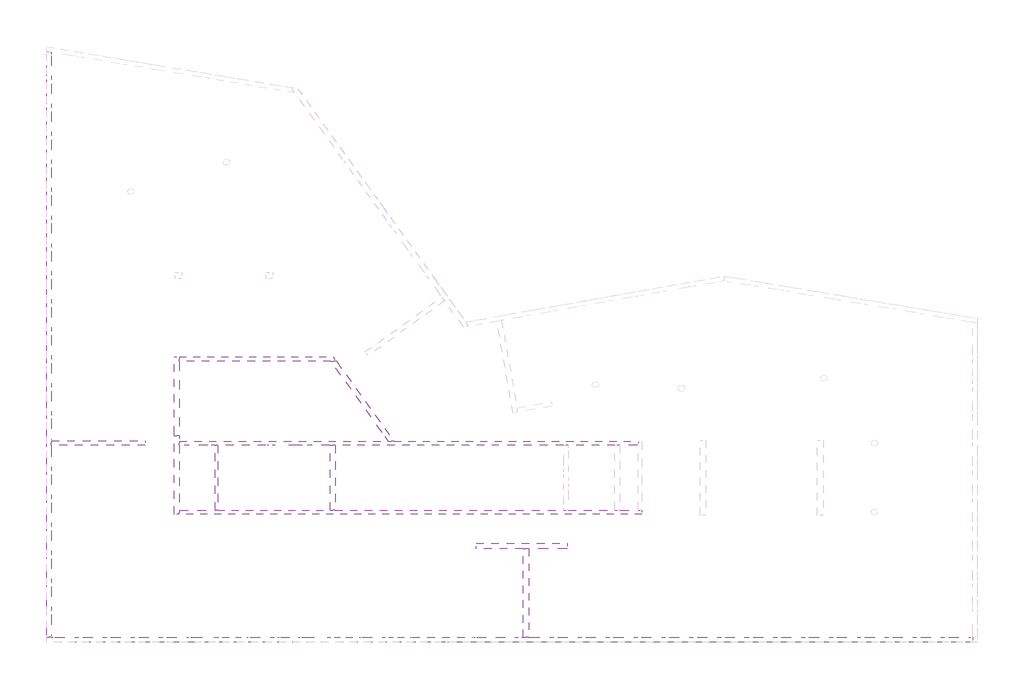
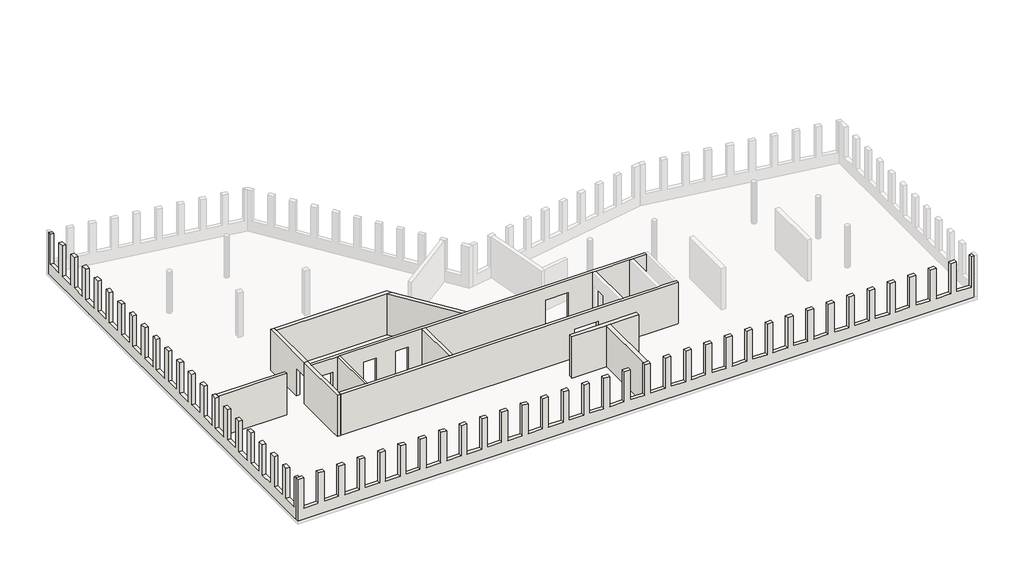
# One storey, part 1 of 2: 13 walls.
"""IFC4 building model written with IfcOpenShell, lengths in millimetres."""

from ifc_helpers import new_model, si_unit, frame, origin, place, context, project, spatial, polyline, outline, extrude, faceted_brep, element, save

model = new_model("IFC4")

# Units and contexts
model_context = context("Model", 3, world=origin())
ifc_project = project(units=[si_unit("LENGTHUNIT", "METRE", prefix="MILLI")], contexts=[model_context])

# Site, building, storey
site = spatial("IfcSite", under=ifc_project)
building = spatial("IfcBuilding", under=site)
storey = spatial("IfcBuildingStorey", under=building, Name="02_OG_OKFB_6,92", Elevation=6920.0)

# Walls
placement = place(None, origin())
element("IfcWall", 1, ObjectType="5dki Lochfassade 26cm C30/37", at=placement, inside=storey, context=model_context, shape_type="Brep", body=[
    faceted_brep([(49396.9999991, 130.0010483, 11090.0), (49396.9999991, 130.0010483, 13440.0), (49603.9991101, 130.0010486, 13440.0), (49603.9991101, 130.0010486, 10230.0), (25766.9999915, 130.0010117, 10230.0), (25466.9999915, 130.0010113, 10230.0), (130.0010047, 130.000972, 10230.0), (-129.9989953, 130.0009716, 10230.0), (-129.9989953, 130.0009716, 13440.0), (130.0010047, 130.000972, 13440.0), (317.0000012, 130.0009723, 13440.0), (316.999997, 130.0009723, 11090.0), (1397.0000012, 130.000974, 11090.0), (1397.0000069, 130.000974, 13440.0), (1816.9999991, 130.0009747, 13440.0), (1817.0000028, 130.0009747, 11090.0), (2896.9999991, 130.0009763, 11090.0), (2897.0000017, 130.0009763, 13440.0), (3316.9999991, 130.000977, 13440.0), (3316.9999977, 130.000977, 11090.0), (4396.9999991, 130.0009787, 11090.0), (4396.9999966, 130.0009787, 13440.0), (4816.9999991, 130.0009793, 13440.0), (4816.9999991, 130.0009793, 11090.0), (5896.9999991, 130.000981, 11090.0), (5896.9999991, 130.000981, 13440.0), (6316.9999991, 130.0009816, 13440.0), (6316.9999991, 130.0009816, 11090.0), (7396.9999991, 130.0009833, 11090.0), (7396.9999991, 130.0009833, 13440.0), (7816.9999991, 130.0009839, 13440.0), (7816.9999991, 130.0009839, 11090.0), (8896.9999991, 130.0009856, 11090.0), (8896.9999991, 130.0009856, 13440.0), (9316.9999991, 130.0009863, 13440.0), (9316.9999991, 130.0009863, 11090.0), (10396.9999991, 130.0009879, 11090.0), (10396.9999991, 130.0009879, 13440.0), (10816.9999991, 130.0009886, 13440.0), (10816.9999991, 130.0009886, 11090.0), (11896.9999991, 130.0009903, 11090.0), (11896.9999991, 130.0009903, 13440.0), (12316.9999991, 130.0009909, 13440.0), (12316.9999991, 130.0009909, 11090.0), (13396.9999991, 130.0009926, 11090.0), (13396.9999991, 130.0009926, 13440.0), (13816.9999991, 130.0009932, 13440.0), (13816.9999991, 130.0009932, 11090.0), (14896.9999991, 130.0009949, 11090.0), (14896.9999991, 130.0009949, 13440.0), (15316.9999991, 130.0009956, 13440.0), (15316.9999991, 130.0009956, 11090.0), (16396.9999991, 130.0009972, 11090.0), (16396.9999991, 130.0009972, 13440.0), (16816.9999991, 130.0009979, 13440.0), (16816.9999991, 130.0009979, 11090.0), (17896.9999991, 130.0009996, 11090.0), (17896.9999991, 130.0009996, 13440.0), (18316.9999991, 130.0010002, 13440.0), (18316.9999991, 130.0010002, 11090.0), (19396.9999991, 130.0010019, 11090.0), (19396.9999991, 130.0010019, 13440.0), (19816.9999991, 130.0010025, 13440.0), (19816.9999991, 130.0010025, 11090.0), (20896.9999991, 130.0010042, 11090.0), (20896.9999991, 130.0010042, 13440.0), (21316.9999991, 130.0010048, 13440.0), (21316.9999991, 130.0010048, 11090.0), (22396.9999991, 130.0010065, 11090.0), (22396.9999991, 130.0010065, 13440.0), (22816.9999991, 130.0010072, 13440.0), (22816.9999991, 130.0010072, 11090.0), (23896.9999991, 130.0010088, 11090.0), (23896.9999991, 130.0010088, 13440.0), (24316.9999991, 130.0010095, 13440.0), (24316.9999991, 130.0010095, 11090.0), (25396.9999991, 130.0010112, 11090.0), (25396.9999991, 130.0010112, 13440.0), (25466.9999915, 130.0010113, 13440.0), (25766.9999915, 130.0010117, 13440.0), (25816.9999991, 130.0010118, 13440.0), (25816.9999991, 130.0010118, 11090.0), (26896.9999991, 130.0010135, 11090.0), (26896.9999991, 130.0010135, 13440.0), (27316.9999991, 130.0010141, 13440.0), (27316.9999991, 130.0010141, 11090.0), (28396.9999991, 130.0010158, 11090.0), (28396.9999991, 130.0010158, 13440.0), (28816.9999991, 130.0010165, 13440.0), (28816.9999991, 130.0010165, 11090.0), (29896.9999991, 130.0010181, 11090.0), (29896.9999991, 130.0010181, 13440.0), (30316.9999991, 130.0010188, 13440.0), (30316.9999991, 130.0010188, 11090.0), (31396.9999991, 130.0010205, 11090.0), (31396.9999991, 130.0010205, 13440.0), (31816.9999991, 130.0010211, 13440.0), (31816.9999991, 130.0010211, 11090.0), (32896.9999991, 130.0010228, 11090.0), (32896.9999991, 130.0010228, 13440.0), (33316.9999991, 130.0010234, 13440.0), (33316.9999991, 130.0010234, 11090.0), (34396.9999991, 130.0010251, 11090.0), (34396.9999991, 130.0010251, 13440.0), (34816.9999991, 130.0010258, 13440.0), (34816.9999991, 130.0010258, 11090.0), (35896.9999991, 130.0010274, 11090.0), (35896.9999991, 130.0010274, 13440.0), (36316.9999991, 130.0010281, 13440.0), (36316.9999991, 130.0010281, 11090.0), (37396.9999991, 130.0010297, 11090.0), (37396.9999991, 130.0010297, 13440.0), (37816.9999991, 130.0010304, 13440.0), (37816.9999991, 130.0010304, 11090.0), (38896.9999991, 130.0010321, 11090.0), (38896.9999991, 130.0010321, 13440.0), (39316.9999991, 130.0010327, 13440.0), (39316.9999991, 130.0010327, 11090.0), (40396.9999991, 130.0010344, 11090.0), (40396.9999991, 130.0010344, 13440.0), (40816.9999991, 130.001035, 13440.0), (40816.9999991, 130.001035, 11090.0), (41896.9999991, 130.0010367, 11090.0), (41896.9999991, 130.0010367, 13440.0), (42316.9999991, 130.0010374, 13440.0), (42316.9999991, 130.0010374, 11090.0), (43396.9999991, 130.001039, 11090.0), (43396.9999991, 130.001039, 13440.0), (43816.9999991, 130.0010397, 13440.0), (43816.9999991, 130.0010397, 11090.0), (44896.9999991, 130.0010414, 11090.0), (44896.9999991, 130.0010414, 13440.0), (45316.9999991, 130.001042, 13440.0), (45316.9999991, 130.001042, 11090.0), (46396.9999991, 130.0010437, 11090.0), (46396.9999991, 130.0010437, 13440.0), (46816.9999991, 130.0010443, 13440.0), (46816.9999991, 130.0010443, 11090.0), (47896.9999991, 130.001046, 11090.0), (47896.9999991, 130.001046, 13440.0), (48316.9999991, 130.0010467, 13440.0), (48316.9999991, 130.0010467, 11090.0), (49603.9991105, -129.9989514, 13440.0), (49396.9999995, -129.9989517, 13440.0), (49396.9999995, -129.9989517, 11090.0), (48316.9999995, -129.9989533, 11090.0), (48316.9999995, -129.9989533, 13440.0), (47896.9999995, -129.998954, 13440.0), (47896.9999995, -129.998954, 11090.0), (46816.9999995, -129.9989557, 11090.0), (46816.9999995, -129.9989557, 13440.0), (46396.9999995, -129.9989563, 13440.0), (46396.9999995, -129.9989563, 11090.0), (45316.9999995, -129.998958, 11090.0), (45316.9999995, -129.998958, 13440.0), (44896.9999995, -129.9989586, 13440.0), (44896.9999995, -129.9989586, 11090.0), (43816.9999995, -129.9989603, 11090.0), (43816.9999995, -129.9989603, 13440.0), (43396.9999995, -129.998961, 13440.0), (43396.9999995, -129.998961, 11090.0), (42316.9999995, -129.9989626, 11090.0), (42316.9999995, -129.9989626, 13440.0), (41896.9999995, -129.9989633, 13440.0), (41896.9999995, -129.9989633, 11090.0), (40816.9999995, -129.998965, 11090.0), (40816.9999995, -129.998965, 13440.0), (40396.9999995, -129.9989656, 13440.0), (40396.9999995, -129.9989656, 11090.0), (39316.9999995, -129.9989673, 11090.0), (39316.9999995, -129.9989673, 13440.0), (38896.9999995, -129.9989679, 13440.0), (38896.9999995, -129.9989679, 11090.0), (37816.9999995, -129.9989696, 11090.0), (37816.9999995, -129.9989696, 13440.0), (37396.9999995, -129.9989703, 13440.0), (37396.9999995, -129.9989703, 11090.0), (36316.9999995, -129.9989719, 11090.0), (36316.9999995, -129.9989719, 13440.0), (35896.9999995, -129.9989726, 13440.0), (35896.9999995, -129.9989726, 11090.0), (34816.9999995, -129.9989742, 11090.0), (34816.9999995, -129.9989742, 13440.0), (34396.9999995, -129.9989749, 13440.0), (34396.9999995, -129.9989749, 11090.0), (33316.9999995, -129.9989766, 11090.0), (33316.9999995, -129.9989766, 13440.0), (32896.9999995, -129.9989772, 13440.0), (32896.9999995, -129.9989772, 11090.0), (31816.9999995, -129.9989789, 11090.0), (31816.9999995, -129.9989789, 13440.0), (31396.9999995, -129.9989795, 13440.0), (31396.9999995, -129.9989795, 11090.0), (30316.9999995, -129.9989812, 11090.0), (30316.9999995, -129.9989812, 13440.0), (29896.9999995, -129.9989819, 13440.0), (29896.9999995, -129.9989819, 11090.0), (28816.9999995, -129.9989835, 11090.0), (28816.9999995, -129.9989835, 13440.0), (28396.9999995, -129.9989842, 13440.0), (28396.9999995, -129.9989842, 11090.0), (27316.9999995, -129.9989859, 11090.0), (27316.9999995, -129.9989859, 13440.0), (26896.9999995, -129.9989865, 13440.0), (26896.9999995, -129.9989865, 11090.0), (25816.9999995, -129.9989882, 11090.0), (25816.9999995, -129.9989882, 13440.0), (25396.9999995, -129.9989888, 13440.0), (25396.9999995, -129.9989888, 11090.0), (24316.9999995, -129.9989905, 11090.0), (24316.9999995, -129.9989905, 13440.0), (23896.9999995, -129.9989912, 13440.0), (23896.9999995, -129.9989912, 11090.0), (22816.9999995, -129.9989928, 11090.0), (22816.9999995, -129.9989928, 13440.0), (22396.9999995, -129.9989935, 13440.0), (22396.9999995, -129.9989935, 11090.0), (21316.9999995, -129.9989952, 11090.0), (21316.9999995, -129.9989952, 13440.0), (20896.9999995, -129.9989958, 13440.0), (20896.9999995, -129.9989958, 11090.0), (19816.9999995, -129.9989975, 11090.0), (19816.9999995, -129.9989975, 13440.0), (19396.9999995, -129.9989981, 13440.0), (19396.9999995, -129.9989981, 11090.0), (18316.9999995, -129.9989998, 11090.0), (18316.9999995, -129.9989998, 13440.0), (17896.9999995, -129.9990004, 13440.0), (17896.9999995, -129.9990004, 11090.0), (16816.9999995, -129.9990021, 11090.0), (16816.9999995, -129.9990021, 13440.0), (16396.9999995, -129.9990028, 13440.0), (16396.9999995, -129.9990028, 11090.0), (15316.9999995, -129.9990044, 11090.0), (15316.9999995, -129.9990044, 13440.0), (14896.9999995, -129.9990051, 13440.0), (14896.9999995, -129.9990051, 11090.0), (13816.9999995, -129.9990068, 11090.0), (13816.9999995, -129.9990068, 13440.0), (13396.9999995, -129.9990074, 13440.0), (13396.9999995, -129.9990074, 11090.0), (12316.9999995, -129.9990091, 11090.0), (12316.9999995, -129.9990091, 13440.0), (11896.9999995, -129.9990097, 13440.0), (11896.9999995, -129.9990097, 11090.0), (10816.9999995, -129.9990114, 11090.0), (10816.9999995, -129.9990114, 13440.0), (10396.9999995, -129.9990121, 13440.0), (10396.9999995, -129.9990121, 11090.0), (9316.9999995, -129.9990137, 11090.0), (9316.9999995, -129.9990137, 13440.0), (8896.9999995, -129.9990144, 13440.0), (8896.9999995, -129.9990144, 11090.0), (7816.9999995, -129.9990161, 11090.0), (7816.9999995, -129.9990161, 13440.0), (7396.9999995, -129.9990167, 13440.0), (7396.9999995, -129.9990167, 11090.0), (6316.9999995, -129.9990184, 11090.0), (6316.9999995, -129.9990184, 13440.0), (5896.9999995, -129.999019, 13440.0), (5896.9999995, -129.999019, 11090.0), (4816.9999995, -129.9990207, 11090.0), (4816.9999995, -129.9990207, 13440.0), (4396.9999995, -129.9990213, 13440.0), (4396.9999966, -129.9990213, 11090.0), (3316.9999995, -129.999023, 11090.0), (3316.9999977, -129.999023, 13440.0), (2896.9999995, -129.9990237, 13440.0), (2897.0000017, -129.9990237, 11090.0), (1816.9999995, -129.9990253, 11090.0), (1817.0000028, -129.9990253, 13440.0), (1397.0000016, -129.999026, 13440.0), (1397.0000069, -129.999026, 11090.0), (317.0000016, -129.9990277, 11090.0), (316.999997, -129.9990277, 13440.0), (-129.9989953, -129.9990284, 13440.0), (-129.9989953, -129.9990284, 10230.0), (49603.9991105, -129.9989514, 10230.0)], [[[0, 1, 2, 3, 4, 5, 6, 7, 8, 9, 10, 11, 12, 13, 14, 15, 16, 17, 18, 19, 20, 21, 22, 23, 24, 25, 26, 27, 28, 29, 30, 31, 32, 33, 34, 35, 36, 37, 38, 39, 40, 41, 42, 43, 44, 45, 46, 47, 48, 49, 50, 51, 52, 53, 54, 55, 56, 57, 58, 59, 60, 61, 62, 63, 64, 65, 66, 67, 68, 69, 70, 71, 72, 73, 74, 75, 76, 77, 78, 79, 80, 81, 82, 83, 84, 85, 86, 87, 88, 89, 90, 91, 92, 93, 94, 95, 96, 97, 98, 99, 100, 101, 102, 103, 104, 105, 106, 107, 108, 109, 110, 111, 112, 113, 114, 115, 116, 117, 118, 119, 120, 121, 122, 123, 124, 125, 126, 127, 128, 129, 130, 131, 132, 133, 134, 135, 136, 137, 138, 139, 140, 141]], [[142, 143, 144, 145, 146, 147, 148, 149, 150, 151, 152, 153, 154, 155, 156, 157, 158, 159, 160, 161, 162, 163, 164, 165, 166, 167, 168, 169, 170, 171, 172, 173, 174, 175, 176, 177, 178, 179, 180, 181, 182, 183, 184, 185, 186, 187, 188, 189, 190, 191, 192, 193, 194, 195, 196, 197, 198, 199, 200, 201, 202, 203, 204, 205, 206, 207, 208, 209, 210, 211, 212, 213, 214, 215, 216, 217, 218, 219, 220, 221, 222, 223, 224, 225, 226, 227, 228, 229, 230, 231, 232, 233, 234, 235, 236, 237, 238, 239, 240, 241, 242, 243, 244, 245, 246, 247, 248, 249, 250, 251, 252, 253, 254, 255, 256, 257, 258, 259, 260, 261, 262, 263, 264, 265, 266, 267, 268, 269, 270, 271, 272, 273, 274, 275, 276, 277]], [[7, 6, 5, 4, 3, 277, 276]], [[17, 267, 266, 18]], [[270, 14, 13, 271]], [[263, 262, 22, 21]], [[259, 258, 26, 25]], [[255, 254, 30, 29]], [[251, 250, 34, 33]], [[247, 246, 38, 37]], [[243, 242, 42, 41]], [[239, 238, 46, 45]], [[235, 234, 50, 49]], [[231, 230, 54, 53]], [[227, 226, 58, 57]], [[223, 222, 62, 61]], [[219, 218, 66, 65]], [[215, 214, 70, 69]], [[211, 210, 74, 73]], [[207, 206, 80, 79, 78, 77]], [[203, 202, 84, 83]], [[199, 198, 88, 87]], [[195, 194, 92, 91]], [[191, 190, 96, 95]], [[187, 186, 100, 99]], [[183, 182, 104, 103]], [[179, 178, 108, 107]], [[175, 174, 112, 111]], [[171, 170, 116, 115]], [[167, 166, 120, 119]], [[163, 162, 124, 123]], [[159, 158, 128, 127]], [[155, 154, 132, 131]], [[151, 150, 136, 135]], [[140, 139, 147, 146]], [[2, 1, 143, 142]], [[10, 9, 8, 275, 274]], [[3, 2, 142, 277]], [[12, 272, 271, 13]], [[273, 11, 10, 274]], [[272, 12, 11, 273]], [[16, 268, 267, 17]], [[269, 15, 14, 270]], [[268, 16, 15, 269]], [[20, 264, 263, 21]], [[265, 19, 18, 266]], [[264, 20, 19, 265]], [[25, 24, 260, 259]], [[23, 22, 262, 261]], [[24, 23, 261, 260]], [[29, 28, 256, 255]], [[27, 26, 258, 257]], [[28, 27, 257, 256]], [[33, 32, 252, 251]], [[31, 30, 254, 253]], [[32, 31, 253, 252]], [[37, 36, 248, 247]], [[35, 34, 250, 249]], [[36, 35, 249, 248]], [[41, 40, 244, 243]], [[39, 38, 246, 245]], [[40, 39, 245, 244]], [[45, 44, 240, 239]], [[43, 42, 242, 241]], [[44, 43, 241, 240]], [[49, 48, 236, 235]], [[47, 46, 238, 237]], [[48, 47, 237, 236]], [[53, 52, 232, 231]], [[51, 50, 234, 233]], [[52, 51, 233, 232]], [[57, 56, 228, 227]], [[55, 54, 230, 229]], [[56, 55, 229, 228]], [[61, 60, 224, 223]], [[59, 58, 226, 225]], [[60, 59, 225, 224]], [[65, 64, 220, 219]], [[63, 62, 222, 221]], [[64, 63, 221, 220]], [[69, 68, 216, 215]], [[67, 66, 218, 217]], [[68, 67, 217, 216]], [[73, 72, 212, 211]], [[71, 70, 214, 213]], [[72, 71, 213, 212]], [[77, 76, 208, 207]], [[75, 74, 210, 209]], [[76, 75, 209, 208]], [[83, 82, 204, 203]], [[81, 80, 206, 205]], [[82, 81, 205, 204]], [[87, 86, 200, 199]], [[85, 84, 202, 201]], [[86, 85, 201, 200]], [[91, 90, 196, 195]], [[89, 88, 198, 197]], [[90, 89, 197, 196]], [[95, 94, 192, 191]], [[93, 92, 194, 193]], [[94, 93, 193, 192]], [[99, 98, 188, 187]], [[97, 96, 190, 189]], [[98, 97, 189, 188]], [[103, 102, 184, 183]], [[101, 100, 186, 185]], [[102, 101, 185, 184]], [[107, 106, 180, 179]], [[105, 104, 182, 181]], [[106, 105, 181, 180]], [[111, 110, 176, 175]], [[109, 108, 178, 177]], [[110, 109, 177, 176]], [[115, 114, 172, 171]], [[113, 112, 174, 173]], [[114, 113, 173, 172]], [[119, 118, 168, 167]], [[117, 116, 170, 169]], [[118, 117, 169, 168]], [[123, 122, 164, 163]], [[121, 120, 166, 165]], [[122, 121, 165, 164]], [[127, 126, 160, 159]], [[125, 124, 162, 161]], [[126, 125, 161, 160]], [[131, 130, 156, 155]], [[129, 128, 158, 157]], [[130, 129, 157, 156]], [[135, 134, 152, 151]], [[133, 132, 154, 153]], [[134, 133, 153, 152]], [[139, 138, 148, 147]], [[137, 136, 150, 149]], [[138, 137, 149, 148]], [[146, 145, 141, 140]], [[144, 143, 1, 0]], [[145, 144, 0, 141]], [[8, 7, 276, 275]]]),
])
element("IfcWall", 2, ObjectType="5dki STB-Wand Kern 25cm C30/37", at=placement, inside=storey, context=model_context, shape_type="Brep", body=[
    faceted_brep([(6989.9999766, 15192.0124447, 13440.0), (6989.9999766, 14942.0124447, 13440.0), (6989.9999766, 10947.0136187, 13440.0), (6989.9999766, 10947.0136187, 12365.0), (6989.9999766, 11957.013616, 12365.0), (6989.9999766, 11957.013616, 10230.0), (6989.9999766, 14942.0124447, 10230.0), (6989.9999766, 15192.0124447, 10230.0), (6739.9999766, 10947.0136187, 13440.0), (6739.9999766, 15192.0124447, 13440.0), (6739.9999766, 15192.0124447, 10230.0), (6739.9999766, 11957.013616, 10230.0), (6739.9999766, 11957.013616, 12365.0), (6739.9999766, 10947.0136187, 12365.0)], [[[0, 1, 2, 3, 4, 5, 6, 7]], [[8, 9, 10, 11, 12, 13]], [[10, 7, 6, 5, 11]], [[2, 1, 0, 9, 8]], [[2, 8, 13, 3]], [[0, 7, 10, 9]], [[4, 12, 11, 5]], [[12, 4, 3, 13]]]),
])
element("IfcWall", 3, ObjectType="5dki STB-Wand Kern 25cm C30/37", at=placement, inside=storey, context=model_context, shape_type="Brep", body=[
    faceted_brep([(6989.9999766, 14942.0124447, 10230.0), (15141.8279932, 14942.0124447, 10230.0), (15449.8792779, 14942.0124447, 10230.0), (15449.8792779, 14942.0124447, 13440.0), (15141.8279932, 14942.0124447, 13440.0), (6989.9999766, 14942.0124447, 13440.0), (6989.9999766, 15192.0124447, 10230.0), (6989.9999766, 15192.0124447, 13440.0), (15269.8915173, 15192.0124447, 13440.0), (15269.8915173, 15192.0124447, 10230.0)], [[[0, 1, 2, 3, 4, 5]], [[6, 7, 8, 9]], [[2, 1, 0, 6, 9]], [[5, 4, 3, 8, 7]], [[0, 5, 7, 6]], [[3, 2, 9, 8]]]),
])
element("IfcWall", 4, ObjectType="5dki STB-Wand Kern 25cm C30/37", at=placement, inside=storey, context=model_context, shape_type="Brep", body=[
    faceted_brep([(18223.2182524, 10662.0127257, 13440.0), (15141.8279932, 14942.0124447, 13440.0), (15141.8279932, 14942.0124447, 10230.0), (17305.3310134, 11936.9428041, 10230.0), (17305.3310134, 11936.9428041, 12365.0), (17895.4523577, 11117.2740911, 12365.0), (17895.4523577, 11117.2740911, 10230.0), (18223.2182524, 10662.0127257, 10230.0), (15449.8792779, 14942.0124447, 13440.0), (18531.2695366, 10662.0127262, 13440.0), (18531.2695366, 10662.0127262, 10230.0), (18098.340653, 11263.3437308, 10230.0), (18098.340653, 11263.3437308, 12365.0), (17508.2193087, 12083.0124438, 12365.0), (17508.2193087, 12083.0124438, 10230.0), (15449.8792779, 14942.0124447, 10230.0)], [[[0, 1, 2, 3, 4, 5, 6, 7]], [[8, 9, 10, 11, 12, 13, 14, 15]], [[2, 15, 14, 3]], [[10, 7, 6, 11]], [[1, 0, 9, 8]], [[2, 1, 8, 15]], [[0, 7, 10, 9]], [[13, 4, 3, 14]], [[4, 13, 12, 5]], [[5, 12, 11, 6]]]),
])
element("IfcWall", 5, ObjectType="5dki STB-Wand Kern 25cm C30/37", at=placement, inside=storey, context=model_context, shape_type="Brep", body=[
    faceted_brep([(6739.9995723, 10947.0136187, 10230.0), (6739.9995723, 6740.0000204, 10230.0), (6739.9995723, 6740.0000204, 13440.0), (6739.9995723, 10947.0136187, 13440.0), (6739.9995723, 10947.0136187, 12365.0), (6989.9995723, 10947.0136187, 10230.0), (6989.9995723, 10947.0136187, 12365.0), (6989.9995723, 10947.0136187, 13440.0), (6989.9995723, 10662.0127052, 13440.0), (6989.9995723, 10442.0127052, 13440.0), (6989.9995723, 6960.0000208, 13440.0), (6989.9995723, 6740.0000208, 13440.0), (6989.9995723, 6740.0000208, 10230.0), (6989.9995723, 6960.0000208, 10230.0), (6989.9995723, 10442.0127052, 10230.0), (6989.9995723, 10662.0127052, 10230.0)], [[[0, 1, 2, 3, 4]], [[5, 6, 7, 8, 9, 10, 11, 12, 13, 14, 15]], [[1, 0, 5, 15, 14, 13, 12]], [[3, 2, 11, 10, 9, 8, 7]], [[0, 4, 3, 7, 6, 5]], [[2, 1, 12, 11]]]),
])
element("IfcWall", 6, ObjectType="5dki STB-Wand Kern 22cm C30/37", at=placement, inside=storey, context=model_context, shape_type="Brep", body=[
    faceted_brep([(31841.999935, 6740.0000516, 13440.0), (6989.9995723, 6740.0000208, 13440.0), (6989.9995723, 6740.0000208, 10230.0), (24166.9999591, 6740.0000421, 10230.0), (24166.999888, 6740.0000421, 12490.0), (25926.9999591, 6740.0000443, 12490.0), (25927.000338, 6740.0000443, 10230.0), (31841.999935, 6740.0000516, 10230.0), (6989.9995723, 6960.0000208, 13440.0), (8916.9999886, 6960.0000232, 13440.0), (9066.9999886, 6960.0000233, 13440.0), (15117.0008797, 6960.0000309, 13440.0), (15367.0008797, 6960.0000312, 13440.0), (27641.9999886, 6960.0000464, 13440.0), (27891.9999886, 6960.0000467, 13440.0), (30391.9999891, 6960.0000498, 13440.0), (30641.9999891, 6960.0000501, 13440.0), (31641.9999382, 6960.0000514, 13440.0), (31841.9999382, 6960.0000516, 13440.0), (31841.9999382, 6960.0000516, 10230.0), (31641.9999382, 6960.0000514, 10230.0), (30641.9999891, 6960.0000501, 10230.0), (30391.9999891, 6960.0000498, 10230.0), (27891.9999886, 6960.0000467, 10230.0), (27641.9999886, 6960.0000464, 10230.0), (25926.9999588, 6960.0000443, 10230.0), (25927.000338, 6960.0000443, 12490.0), (24166.9999588, 6960.0000421, 12490.0), (24166.999888, 6960.0000421, 10230.0), (15367.0008797, 6960.0000312, 10230.0), (15117.0008797, 6960.0000309, 10230.0), (9066.9999886, 6960.0000233, 10230.0), (8916.9999886, 6960.0000232, 10230.0), (6989.9995723, 6960.0000208, 10230.0)], [[[0, 1, 2, 3, 4, 5, 6, 7]], [[8, 9, 10, 11, 12, 13, 14, 15, 16, 17, 18, 19, 20, 21, 22, 23, 24, 25, 26, 27, 28, 29, 30, 31, 32, 33]], [[2, 33, 32, 31, 30, 29, 28, 3]], [[19, 7, 6, 25, 24, 23, 22, 21, 20]], [[1, 0, 18, 17, 16, 15, 14, 13, 12, 11, 10, 9, 8]], [[2, 1, 8, 33]], [[0, 7, 19, 18]], [[5, 26, 25, 6]], [[26, 5, 4, 27]], [[27, 4, 3, 28]]]),
])
element("IfcWall", 7, ObjectType="5dki STB-Wand Kern 22cm C30/37", at=placement, inside=storey, context=model_context, shape_type="Brep", body=[
    faceted_brep([(6989.9995723, 10662.0127052, 13440.0), (18223.2182524, 10662.0127257, 13440.0), (18531.2695366, 10662.0127262, 13440.0), (31641.9999912, 10662.0127502, 13440.0), (31641.9999912, 10662.0127502, 10230.0), (25926.999945, 10662.0127397, 10230.0), (25927.0000254, 10662.0127397, 12490.0), (24166.999945, 10662.0127365, 12490.0), (24166.9998144, 10662.0127365, 10230.0), (18531.2695366, 10662.0127262, 10230.0), (18223.2182524, 10662.0127257, 10230.0), (14152.0004935, 10662.0127182, 10230.0), (14152.0007698, 10662.0127182, 12365.0), (13142.0004935, 10662.0127164, 12365.0), (13142.0009721, 10662.0127164, 10230.0), (11796.9999806, 10662.0127139, 10230.0), (11796.9997327, 10662.0127139, 12365.0), (10786.9999806, 10662.0127121, 12365.0), (10786.999935, 10662.0127121, 10230.0), (8540.0010342, 10662.012708, 10230.0), (8540.000485, 10662.012708, 12365.0), (7530.0010342, 10662.0127061, 12365.0), (7530.0006873, 10662.0127061, 10230.0), (6989.9995723, 10662.0127052, 10230.0), (31641.9999881, 10442.0127502, 13440.0), (30641.9999891, 10442.0127483, 13440.0), (30391.9999891, 10442.0127479, 13440.0), (27891.9999829, 10442.0127433, 13440.0), (27641.9999829, 10442.0127429, 13440.0), (15367.0008797, 10442.0127204, 13440.0), (15117.0008797, 10442.01272, 13440.0), (9066.9999886, 10442.0127089, 13440.0), (8916.9999886, 10442.0127087, 13440.0), (6989.9995723, 10442.0127052, 13440.0), (6989.9995723, 10442.0127052, 10230.0), (7530.0010346, 10442.0127061, 10230.0), (7530.0006873, 10442.0127061, 12365.0), (8540.0010346, 10442.012708, 12365.0), (8540.000485, 10442.012708, 10230.0), (8916.9999886, 10442.0127087, 10230.0), (9066.9999886, 10442.0127089, 10230.0), (10786.999981, 10442.0127121, 10230.0), (10786.999935, 10442.0127121, 12365.0), (11796.999981, 10442.0127139, 12365.0), (11796.9997327, 10442.0127139, 10230.0), (13142.0004939, 10442.0127164, 10230.0), (13142.0009721, 10442.0127164, 12365.0), (14152.0004939, 10442.0127182, 12365.0), (14152.0007698, 10442.0127182, 10230.0), (15117.0008797, 10442.01272, 10230.0), (15367.0008797, 10442.0127204, 10230.0), (24166.9999454, 10442.0127365, 10230.0), (24166.9998144, 10442.0127365, 12490.0), (25926.9999454, 10442.0127397, 12490.0), (25927.0000254, 10442.0127397, 10230.0), (27641.9999829, 10442.0127429, 10230.0), (27891.9999829, 10442.0127433, 10230.0), (30391.9999891, 10442.0127479, 10230.0), (30641.9999891, 10442.0127483, 10230.0), (31641.9999881, 10442.0127502, 10230.0)], [[[0, 1, 2, 3, 4, 5, 6, 7, 8, 9, 10, 11, 12, 13, 14, 15, 16, 17, 18, 19, 20, 21, 22, 23]], [[24, 25, 26, 27, 28, 29, 30, 31, 32, 33, 34, 35, 36, 37, 38, 39, 40, 41, 42, 43, 44, 45, 46, 47, 48, 49, 50, 51, 52, 53, 54, 55, 56, 57, 58, 59]], [[34, 23, 22, 35]], [[4, 59, 58, 57, 56, 55, 54, 5]], [[8, 51, 50, 49, 48, 11, 10, 9]], [[18, 41, 40, 39, 38, 19]], [[44, 15, 14, 45]], [[3, 2, 1, 0, 33, 32, 31, 30, 29, 28, 27, 26, 25, 24]], [[0, 23, 34, 33]], [[4, 3, 24, 59]], [[53, 6, 5, 54]], [[6, 53, 52, 7]], [[7, 52, 51, 8]], [[17, 42, 41, 18]], [[42, 17, 16, 43]], [[43, 16, 15, 44]], [[13, 46, 45, 14]], [[46, 13, 12, 47]], [[47, 12, 11, 48]], [[21, 36, 35, 22]], [[36, 21, 20, 37]], [[37, 20, 19, 38]]]),
])
element("IfcWall", 8, ObjectType="5dki STB-Wand Kern 25cm C30/37", at=placement, inside=storey, context=model_context, shape_type="SweptSolid", body=[
    extrude(outline(polyline([(15117.0008797, 6960.0000309), (15117.0008797, 10442.01272), (15367.0008797, 10442.0127204), (15367.0008797, 6960.0000312), (15117.0008797, 6960.0000309)])), frame((0.0, 0.0, 10230.0), z_axis=(0.0, 0.0, 1.0), x_axis=(1.0, 0.0, 0.0)), (0.0, 0.0, 1.0), 3210.0),
])
element("IfcWall", 9, ObjectType="5dki STB-Wand Kern 15cm C30/37", at=placement, inside=storey, context=model_context, shape_type="SweptSolid", body=[
    extrude(outline(polyline([(8916.9999886, 6960.0000232), (8916.9999886, 10442.0127087), (9066.9999886, 10442.0127089), (9066.9999886, 6960.0000233), (8916.9999886, 6960.0000232)])), frame((0.0, 0.0, 10230.0), z_axis=(0.0, 0.0, 1.0), x_axis=(1.0, 0.0, 0.0)), (0.0, 0.0, 1.0), 3210.0),
])
element("IfcWall", 10, ObjectType="5dki Lochfassade 26cm C30/37", at=placement, inside=storey, context=model_context, shape_type="Brep", body=[
    faceted_brep([(130.0010047, 24278.4322867, 11090.0), (130.0010047, 24278.4322867, 13440.0), (130.0010047, 23857.0124158, 13440.0), (130.0010047, 23857.0124158, 11090.0), (130.0010047, 22777.0124158, 11090.0), (130.0010047, 22777.0124158, 13440.0), (130.0010047, 22357.0124158, 13440.0), (130.0010047, 22357.0124158, 11090.0), (130.0010047, 21277.0124158, 11090.0), (130.0010047, 21277.0124158, 13440.0), (130.0010047, 20857.0124158, 13440.0), (130.0010047, 20857.0124158, 11090.0), (130.0010047, 19777.0124158, 11090.0), (130.0010047, 19777.0124158, 13440.0), (130.0010047, 19357.0124158, 13440.0), (130.0010047, 19357.0124158, 11090.0), (130.0010047, 18277.0124158, 11090.0), (130.0010047, 18277.0124158, 13440.0), (130.0010047, 17857.0124158, 13440.0), (130.0010047, 17857.0124158, 11090.0), (130.0010047, 16777.0124158, 11090.0), (130.0010047, 16777.0124158, 13440.0), (130.0010047, 16357.0124158, 13440.0), (130.0010047, 16357.0124158, 11090.0), (130.0010047, 15277.0124158, 11090.0), (130.0010047, 15277.0124158, 13440.0), (130.0010047, 14857.0124158, 13440.0), (130.0010047, 14857.0124158, 11090.0), (130.0010047, 13777.0124158, 11090.0), (130.0010047, 13777.0124158, 13440.0), (130.0010047, 13357.0124158, 13440.0), (130.0010047, 13357.0124158, 11090.0), (130.0010047, 12277.0124158, 11090.0), (130.0010047, 12277.0124158, 13440.0), (130.0010047, 11857.0124158, 13440.0), (130.0010047, 11857.0124158, 11090.0), (130.0010047, 10777.0124158, 11090.0), (130.0010047, 10777.0124158, 13440.0), (130.0010047, 10692.0124295, 13440.0), (130.0010047, 10442.0124295, 13440.0), (130.0010047, 10357.0124158, 13440.0), (130.0010047, 10357.0124158, 11090.0), (130.0010047, 9277.0124158, 11090.0), (130.0010047, 9277.0124158, 13440.0), (130.0010047, 8857.0124158, 13440.0), (130.0010047, 8857.0124158, 11090.0), (130.0010047, 7777.0124158, 11090.0), (130.0010047, 7777.0124158, 13440.0), (130.0010047, 7357.0124158, 13440.0), (130.0010047, 7357.0124158, 11090.0), (130.0010047, 6277.0124158, 11090.0), (130.0010047, 6277.0124158, 13440.0), (130.0010047, 5857.0124158, 13440.0), (130.0010047, 5857.0124158, 11090.0), (130.0010047, 4777.0124158, 11090.0), (130.0010047, 4777.0124158, 13440.0), (130.0010047, 4357.0124158, 13440.0), (130.0010047, 4357.0124158, 11090.0), (130.0010047, 3277.0124158, 11090.0), (130.0010047, 3277.0124158, 13440.0), (130.0010047, 2857.0124158, 13440.0), (130.0010047, 2857.0124158, 11090.0), (130.0010047, 1777.0124158, 11090.0), (130.0010047, 1777.0124158, 13440.0), (130.0010047, 1357.0124158, 13440.0), (130.0010047, 1357.0124158, 11090.0), (130.0010047, 277.0124158, 11090.0), (130.0010047, 277.0124158, 13440.0), (130.0010047, 130.000972, 13440.0), (130.0010047, 130.000972, 10230.0), (130.0010047, 10442.0124295, 10230.0), (130.0010047, 10692.0124295, 10230.0), (130.0010047, 31548.6978518, 10230.0), (130.0010047, 31548.6978518, 13440.0), (130.0010047, 31357.0124158, 13440.0), (130.0010047, 31357.0124158, 11090.0), (130.0010047, 30277.0124158, 11090.0), (130.0010047, 30277.0124158, 13440.0), (130.0010047, 29857.0124158, 13440.0), (130.0010047, 29857.0124158, 11090.0), (130.0010047, 28777.0124158, 11090.0), (130.0010047, 28777.0124158, 13440.0), (130.0010047, 28358.4322867, 13440.0), (130.0010047, 28358.4322867, 11090.0), (130.0010047, 27278.4322867, 11090.0), (130.0010047, 27278.4322867, 13440.0), (130.0010047, 26858.4322867, 13440.0), (130.0010047, 26858.4322867, 11090.0), (130.0010047, 25778.4322867, 11090.0), (130.0010047, 25778.4322867, 13440.0), (130.0010047, 25358.4322867, 13440.0), (130.0010047, 25358.4322867, 11090.0), (-129.9989953, 23857.0124158, 13440.0), (-129.9989953, 24278.4322867, 13440.0), (-129.9989953, 24278.4322867, 11090.0), (-129.9989953, 25358.4322867, 11090.0), (-129.9989953, 25358.4322867, 13440.0), (-129.9989953, 25778.4322867, 13440.0), (-129.9989953, 25778.4322867, 11090.0), (-129.9989953, 26858.4322867, 11090.0), (-129.9989953, 26858.4322867, 13440.0), (-129.9989953, 27278.4322867, 13440.0), (-129.9989953, 27278.4322867, 11090.0), (-129.9989953, 28358.4322867, 11090.0), (-129.9989953, 28358.4322867, 13440.0), (-129.9989953, 28777.0124158, 13440.0), (-129.9989953, 28777.0124158, 11090.0), (-129.9989953, 29857.0124158, 11090.0), (-129.9989953, 29857.0124158, 13440.0), (-129.9989953, 30277.0124158, 13440.0), (-129.9989953, 30277.0124158, 11090.0), (-129.9989953, 31357.0124158, 11090.0), (-129.9989953, 31357.0124158, 13440.0), (-129.9989953, 31592.114918, 13440.0), (-129.9989953, 31592.114918, 10230.0), (-129.9989953, 130.0009716, 10230.0), (-129.9989953, 130.0009716, 13440.0), (-129.9989953, 277.0124158, 13440.0), (-129.9989953, 277.0124158, 11090.0), (-129.9989953, 1357.0124158, 11090.0), (-129.9989953, 1357.0124158, 13440.0), (-129.9989953, 1777.0124158, 13440.0), (-129.9989953, 1777.0124158, 11090.0), (-129.9989953, 2857.0124158, 11090.0), (-129.9989953, 2857.0124158, 13440.0), (-129.9989953, 3277.0124158, 13440.0), (-129.9989953, 3277.0124158, 11090.0), (-129.9989953, 4357.0124158, 11090.0), (-129.9989953, 4357.0124158, 13440.0), (-129.9989953, 4777.0124158, 13440.0), (-129.9989953, 4777.0124158, 11090.0), (-129.9989953, 5857.0124158, 11090.0), (-129.9989953, 5857.0124158, 13440.0), (-129.9989953, 6277.0124158, 13440.0), (-129.9989953, 6277.0124158, 11090.0), (-129.9989953, 7357.0124158, 11090.0), (-129.9989953, 7357.0124158, 13440.0), (-129.9989953, 7777.0124158, 13440.0), (-129.9989953, 7777.0124158, 11090.0), (-129.9989953, 8857.0124158, 11090.0), (-129.9989953, 8857.0124158, 13440.0), (-129.9989953, 9277.0124158, 13440.0), (-129.9989953, 9277.0124158, 11090.0), (-129.9989953, 10357.0124158, 11090.0), (-129.9989953, 10357.0124158, 13440.0), (-129.9989953, 10777.0124158, 13440.0), (-129.9989953, 10777.0124158, 11090.0), (-129.9989953, 11857.0124158, 11090.0), (-129.9989953, 11857.0124158, 13440.0), (-129.9989953, 12277.0124158, 13440.0), (-129.9989953, 12277.0124158, 11090.0), (-129.9989953, 13357.0124158, 11090.0), (-129.9989953, 13357.0124158, 13440.0), (-129.9989953, 13777.0124158, 13440.0), (-129.9989953, 13777.0124158, 11090.0), (-129.9989953, 14857.0124158, 11090.0), (-129.9989953, 14857.0124158, 13440.0), (-129.9989953, 15277.0124158, 13440.0), (-129.9989953, 15277.0124158, 11090.0), (-129.9989953, 16357.0124158, 11090.0), (-129.9989953, 16357.0124158, 13440.0), (-129.9989953, 16777.0124158, 13440.0), (-129.9989953, 16777.0124158, 11090.0), (-129.9989953, 17857.0124158, 11090.0), (-129.9989953, 17857.0124158, 13440.0), (-129.9989953, 18277.0124158, 13440.0), (-129.9989953, 18277.0124158, 11090.0), (-129.9989953, 19357.0124158, 11090.0), (-129.9989953, 19357.0124158, 13440.0), (-129.9989953, 19777.0124158, 13440.0), (-129.9989953, 19777.0124158, 11090.0), (-129.9989953, 20857.0124158, 11090.0), (-129.9989953, 20857.0124158, 13440.0), (-129.9989953, 21277.0124158, 13440.0), (-129.9989953, 21277.0124158, 11090.0), (-129.9989953, 22357.0124158, 11090.0), (-129.9989953, 22357.0124158, 13440.0), (-129.9989953, 22777.0124158, 13440.0), (-129.9989953, 22777.0124158, 11090.0), (-129.9989953, 23857.0124158, 11090.0), (90.4211678, 31555.307238, 13440.0)], [[[0, 1, 2, 3, 4, 5, 6, 7, 8, 9, 10, 11, 12, 13, 14, 15, 16, 17, 18, 19, 20, 21, 22, 23, 24, 25, 26, 27, 28, 29, 30, 31, 32, 33, 34, 35, 36, 37, 38, 39, 40, 41, 42, 43, 44, 45, 46, 47, 48, 49, 50, 51, 52, 53, 54, 55, 56, 57, 58, 59, 60, 61, 62, 63, 64, 65, 66, 67, 68, 69, 70, 71, 72, 73, 74, 75, 76, 77, 78, 79, 80, 81, 82, 83, 84, 85, 86, 87, 88, 89, 90, 91]], [[92, 93, 94, 95, 96, 97, 98, 99, 100, 101, 102, 103, 104, 105, 106, 107, 108, 109, 110, 111, 112, 113, 114, 115, 116, 117, 118, 119, 120, 121, 122, 123, 124, 125, 126, 127, 128, 129, 130, 131, 132, 133, 134, 135, 136, 137, 138, 139, 140, 141, 142, 143, 144, 145, 146, 147, 148, 149, 150, 151, 152, 153, 154, 155, 156, 157, 158, 159, 160, 161, 162, 163, 164, 165, 166, 167, 168, 169, 170, 171, 172, 173, 174, 175, 176, 177, 178, 179]], [[72, 71, 70, 69, 115, 114]], [[64, 63, 121, 120]], [[60, 59, 125, 124]], [[56, 55, 129, 128]], [[52, 51, 133, 132]], [[48, 47, 137, 136]], [[44, 43, 141, 140]], [[40, 39, 38, 37, 145, 144]], [[34, 33, 149, 148]], [[30, 29, 153, 152]], [[26, 25, 157, 156]], [[22, 21, 161, 160]], [[18, 17, 165, 164]], [[14, 13, 169, 168]], [[10, 9, 173, 172]], [[6, 5, 177, 176]], [[74, 73, 180, 113, 112]], [[78, 77, 109, 108]], [[82, 81, 105, 104]], [[86, 85, 101, 100]], [[90, 89, 97, 96]], [[2, 1, 93, 92]], [[116, 68, 67, 117]], [[119, 65, 64, 120]], [[66, 118, 117, 67]], [[65, 119, 118, 66]], [[124, 123, 61, 60]], [[122, 121, 63, 62]], [[123, 122, 62, 61]], [[128, 127, 57, 56]], [[126, 125, 59, 58]], [[127, 126, 58, 57]], [[132, 131, 53, 52]], [[130, 129, 55, 54]], [[131, 130, 54, 53]], [[136, 135, 49, 48]], [[134, 133, 51, 50]], [[135, 134, 50, 49]], [[140, 139, 45, 44]], [[138, 137, 47, 46]], [[139, 138, 46, 45]], [[144, 143, 41, 40]], [[142, 141, 43, 42]], [[143, 142, 42, 41]], [[148, 147, 35, 34]], [[146, 145, 37, 36]], [[147, 146, 36, 35]], [[152, 151, 31, 30]], [[150, 149, 33, 32]], [[151, 150, 32, 31]], [[156, 155, 27, 26]], [[154, 153, 29, 28]], [[155, 154, 28, 27]], [[160, 159, 23, 22]], [[158, 157, 25, 24]], [[159, 158, 24, 23]], [[164, 163, 19, 18]], [[162, 161, 21, 20]], [[163, 162, 20, 19]], [[168, 167, 15, 14]], [[166, 165, 17, 16]], [[167, 166, 16, 15]], [[172, 171, 11, 10]], [[170, 169, 13, 12]], [[171, 170, 12, 11]], [[176, 175, 7, 6]], [[174, 173, 9, 8]], [[175, 174, 8, 7]], [[92, 179, 3, 2]], [[178, 177, 5, 4]], [[179, 178, 4, 3]], [[112, 111, 75, 74]], [[110, 109, 77, 76]], [[111, 110, 76, 75]], [[108, 107, 79, 78]], [[106, 105, 81, 80]], [[107, 106, 80, 79]], [[104, 103, 83, 82]], [[102, 101, 85, 84]], [[103, 102, 84, 83]], [[100, 99, 87, 86]], [[98, 97, 89, 88]], [[99, 98, 88, 87]], [[96, 95, 91, 90]], [[94, 93, 1, 0]], [[95, 94, 0, 91]], [[69, 68, 116, 115]], [[73, 72, 114, 113, 180]]]),
])
element("IfcWall", 11, ObjectType="5dki STB-Wand 25cm C30/37", at=placement, inside=storey, context=model_context, shape_type="SweptSolid", body=[
    extrude(outline(polyline([(130.0010047, 10692.0124295), (5179.9999831, 10692.0124295), (5179.9999831, 10442.0124295), (130.0010047, 10442.0124295), (130.0010047, 10692.0124295)])), frame((0.0, 0.0, 10230.0), z_axis=(0.0, 0.0, 1.0), x_axis=(1.0, 0.0, 0.0)), (0.0, 0.0, 1.0), 3210.0),
])
element("IfcWall", 12, ObjectType="5dki STB-Wand 30cm C30/37", at=placement, inside=storey, context=model_context, shape_type="Brep", body=[
    faceted_brep([(22936.4905033, 4880.0000432, 10230.0), (25466.9999915, 4880.0000432, 10230.0), (25766.9999915, 4880.0000432, 10230.0), (27842.0010332, 4880.0000432, 10230.0), (27842.0010332, 4880.0000432, 13440.0), (25766.9999915, 4880.0000432, 13440.0), (25466.9999915, 4880.0000432, 13440.0), (22936.4905033, 4880.0000432, 13440.0), (22936.4905033, 5180.0000432, 10230.0), (22936.4905033, 5180.0000432, 13440.0), (27842.0010332, 5180.0000432, 13440.0), (27842.0010332, 5180.0000432, 10230.0)], [[[0, 1, 2, 3, 4, 5, 6, 7]], [[8, 9, 10, 11]], [[3, 2, 1, 0, 8, 11]], [[4, 3, 11, 10]], [[7, 6, 5, 4, 10, 9]], [[0, 7, 9, 8]]]),
])
element("IfcWall", 13, ObjectType="5dki STB-Wand 30cm C30/37", at=placement, inside=storey, context=model_context, shape_type="SweptSolid", body=[
    extrude(outline(polyline([(25466.9999915, 130.0010113), (25466.9999915, 4880.0000432), (25766.9999915, 4880.0000432), (25766.9999915, 130.0010117), (25466.9999915, 130.0010113)])), frame((0.0, 0.0, 10230.0), z_axis=(0.0, 0.0, 1.0), x_axis=(1.0, 0.0, 0.0)), (0.0, 0.0, 1.0), 3210.0),
])

save(model, "model.ifc")

# Revit data of these elements
# Type "5dki Lochfassade 26cm C30/37"
#   Type Comments = ""
#   Description = ""
#   cpiComponentType = "Wall"
#   cpiFitMatchKey = "5D-KI-STB-OB-W-LF"
#   5d Materialgüte = "C35/45"
#   Filter Tragend / Nichttragend = yes
#   5dki WU = no
#   Layers, outside or top first: 0.260 m "5d Beton - Stahlbeton" (function 1)
# Type "5dki STB-Wand Kern 25cm C30/37"
#   Type Comments = ""
#   Description = ""
#   cpiComponentType = "Wall"
#   cpiFitMatchKey = "5D-KI-STB-OB-W-K"
#   5d Materialgüte = "C30/37"
#   Filter Tragend / Nichttragend = yes
#   5dki WU = no
#   Layers, outside or top first: 0.250 m "5d Beton - Stahlbeton" (function 1)
# Type "5dki STB-Wand Kern 22cm C30/37"
#   Type Comments = ""
#   Description = ""
#   cpiComponentType = "Wall"
#   cpiFitMatchKey = "5D-KI-STB-OB-W-K"
#   5d Materialgüte = "C30/37"
#   Filter Tragend / Nichttragend = yes
#   5dki WU = no
#   Layers, outside or top first: 0.220 m "5d Beton - Stahlbeton" (function 1)
# Type "5dki STB-Wand Kern 15cm C30/37"
#   Type Comments = ""
#   Description = ""
#   cpiComponentType = "Wall"
#   cpiFitMatchKey = "5D-KI-STB-OB-W-K"
#   5d Materialgüte = "C30/37"
#   Filter Tragend / Nichttragend = yes
#   5dki WU = no
#   Layers, outside or top first: 0.150 m "5d Beton - Stahlbeton" (function 1)
# Type "5dki STB-Wand 25cm C30/37"
#   Type Comments = ""
#   Description = ""
#   cpiComponentType = "Wall"
#   cpiFitMatchKey = "5D-KI-STB-OB-W"
#   5d Materialgüte = "C30/37"
#   Filter Tragend / Nichttragend = yes
#   5dki WU = no
#   Layers, outside or top first: 0.250 m "5d Beton - Stahlbeton" (function 1)
# Type "5dki STB-Wand 30cm C30/37"
#   Type Comments = ""
#   Description = ""
#   cpiComponentType = "Wall"
#   cpiFitMatchKey = "5D-KI-STB-OB-W"
#   5d Materialgüte = "C30/37"
#   Filter Tragend / Nichttragend = yes
#   5dki WU = no
#   Layers, outside or top first: 0.300 m "5d Beton - Stahlbeton" (function 1)
# Element 1 (IfcWall, "5dki Lochfassade 26cm C30/37")
#   000_080_030_Geschoß = "03_OG"
#   Top Offset = 0.000 m
#   Base Offset = 0.000 m
#   wall height = 3.210 m
#   Phase Created = Neu
#   Base Constraint = 02_OG_OKRD_10,23
#   Top Constraint = 03_OG_UKRD_13,44
#   Materials on its faces: "5d Beton - Stahlbeton"
# Elements 2, 3, 4, 5, 8 (IfcWall, "5dki STB-Wand Kern 25cm C30/37")
#   Comments = ""
#   000_080_030_Geschoß = "03_OG"
#   Top Offset = 0.000 m
#   Base Offset = 0.000 m
#   wall height = 3.210 m
#   Phase Created = Neu
#   Base Constraint = 02_OG_OKRD_10,23
#   Top Constraint = 03_OG_UKRD_13,44
#   Materials on its faces: "5d Beton - Stahlbeton"
# Elements 6, 7 (IfcWall, "5dki STB-Wand Kern 22cm C30/37")
#   Comments = ""
#   000_080_030_Geschoß = "03_OG"
#   Top Offset = 0.000 m
#   Base Offset = 0.000 m
#   wall height = 3.210 m
#   Phase Created = Neu
#   Base Constraint = 02_OG_OKRD_10,23
#   Top Constraint = 03_OG_UKRD_13,44
#   Materials on its faces: "5d Beton - Stahlbeton"
# Element 9 (IfcWall, "5dki STB-Wand Kern 15cm C30/37")
#   Comments = ""
#   000_080_030_Geschoß = "03_OG"
#   Top Offset = 0.000 m
#   Base Offset = 0.000 m
#   wall height = 3.210 m
#   Phase Created = Neu
#   Base Constraint = 02_OG_OKRD_10,23
#   Top Constraint = 03_OG_UKRD_13,44
#   Materials on its faces: "5d Beton - Stahlbeton"
# Element 10 (IfcWall, "5dki Lochfassade 26cm C30/37")
#   Comments = ""
#   000_080_030_Geschoß = "03_OG"
#   Top Offset = 0.000 m
#   Base Offset = 0.000 m
#   wall height = 3.210 m
#   Phase Created = Neu
#   Base Constraint = 02_OG_OKRD_10,23
#   Top Constraint = 03_OG_UKRD_13,44
#   Materials on its faces: "5d Beton - Stahlbeton"
# Element 11 (IfcWall, "5dki STB-Wand 25cm C30/37")
#   Comments = ""
#   000_080_030_Geschoß = "03_OG"
#   Top Offset = 0.000 m
#   Base Offset = 0.000 m
#   wall height = 3.210 m
#   Phase Created = Neu
#   Base Constraint = 02_OG_OKRD_10,23
#   Top Constraint = 03_OG_UKRD_13,44
#   Materials on its faces: "5d Beton - Stahlbeton"
# Element 12 (IfcWall, "5dki STB-Wand 30cm C30/37")
#   Comments = ""
#   000_080_030_Geschoß = "03_OG"
#   Top Offset = 0.000 m
#   Base Offset = 0.000 m
#   wall height = 3.210 m
#   Phase Created = Neu
#   Base Constraint = 02_OG_OKRD_10,23
#   Top Constraint = 03_OG_UKRD_13,44
#   Materials on its faces: "5d Beton - Stahlbeton"
# Element 13 (IfcWall, "5dki STB-Wand 30cm C30/37")
#   000_080_030_Geschoß = "03_OG"
#   Top Offset = 0.000 m
#   Base Offset = 0.000 m
#   wall height = 3.210 m
#   Phase Created = Neu
#   Base Constraint = 02_OG_OKRD_10,23
#   Top Constraint = 03_OG_UKRD_13,44
#   Materials on its faces: "5d Beton - Stahlbeton"
# Materials
#   "5d Beton - Stahlbeton": class "5dki", colour RGB 200 200 200, transparency 0, Cost = 0
